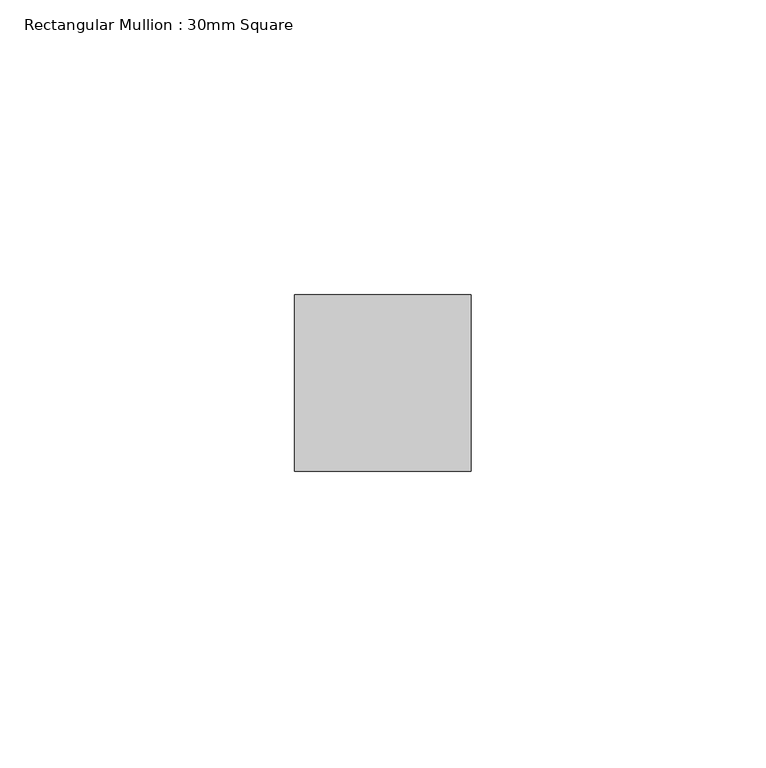
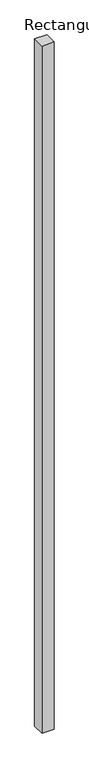
"""IFC4 building model written with IfcOpenShell, lengths in millimetres: member geometry, Rectangular Mullion : 30mm Square."""

from ifc_helpers import new_model, si_unit, frame, origin, place, context, project, spatial, polyline, outline, extrude, source, transform, mapped, element, save


def rectangular_mullion_30mm_square_e1a034c2(model_context):
    return source(origin(), model_context, "Body", "SweptSolid", [
        extrude(outline(polyline([(15.0, 15.0), (15.0, -15.0), (-15.0, -15.0), (-15.0, 15.0), (15.0, 15.0)])), frame((0.0, 0.0, -1769.3235909), z_axis=(0.0, 0.0, 1.0), x_axis=(1.0, 0.0, 0.0)), (0.0, 0.0, 1.0), 1769.3235909),
    ])


if __name__ == "__main__":
    model = new_model("IFC4")
    model_context = context("Model", 3, world=origin())
    ifc_project = project(units=[si_unit("LENGTHUNIT", "METRE", prefix="MILLI")], contexts=[model_context])
    site = spatial("IfcSite", under=ifc_project)
    building = spatial("IfcBuilding", under=site)
    placement = place(None, origin())
    rectangular_mullion_30mm_square_shape = rectangular_mullion_30mm_square_e1a034c2(model_context)
    element("IfcMember", 1, ObjectType="Rectangular Mullion : 30mm Square", at=placement, inside=building, context=model_context, shape_type="MappedRepresentation", body=[
        mapped(rectangular_mullion_30mm_square_shape, transform((0.0, 0.0, 0.0), x_axis=(1.0, 0.0, 0.0), y_axis=(0.0, 1.0, 0.0), z_axis=(0.0, 0.0, 1.0))),
    ])
    save(model, "model.ifc")

# Revit data of these elements
# Type "Rectangular Mullion : 30mm Square"
#   built-in parameter 1007304 = 0.0984252 (stored number, unit not read)
#   built-in parameter 1007301 = 0.0492126 (stored number, unit not read)
#   built-in parameter 1007300 = 0.0492126 (stored number, unit not read)
# Element 1 (IfcMember, "Rectangular Mullion : 30mm Square")
#   Materials on its faces: "Aluminum"
# Materials
#   "Aluminum": class "Metal", colour RGB 244 244 244, transparency 0, Description = "Aluminum 6061", Cost = 0
